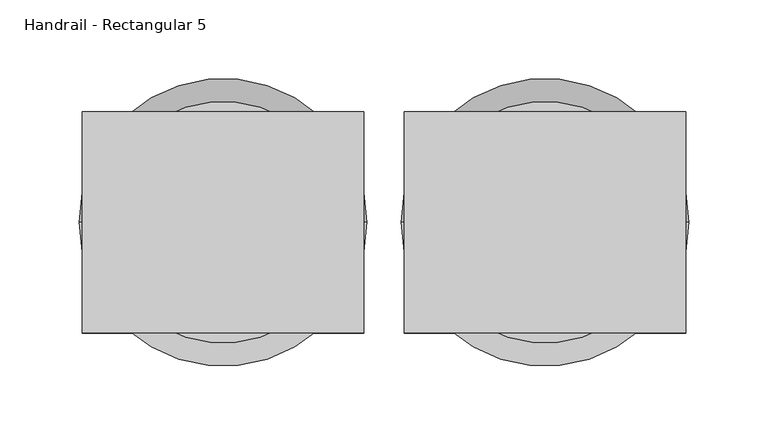
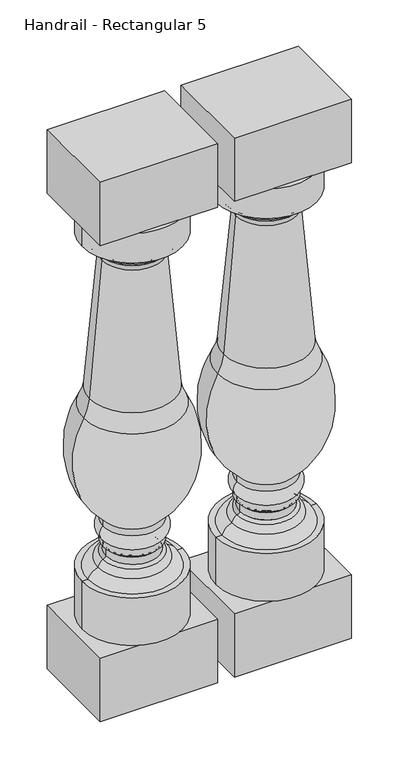
"""IFC4 building model written with IfcOpenShell, lengths in millimetres: railing geometry, Handrail - Rectangular 5."""

from ifc_helpers import new_model, si_unit, point, frame, origin, place, context, project, spatial, polyline, circle_curve, ellipse_curve, trimmed, outline, extrude, source, transform, mapped, element, save
from ifc_brep_helpers import plane_surface, cylinder_surface, revolved_surface, advanced_brep


def handrail_rectangular_5_87bace6c(model_context):
    return source(origin(), model_context, "Body", "SolidModel", [
        advanced_brep(
        [(16901.0521895, -1665.6164768, 873.125), (17053.4521895, -1665.6164768, 873.125), (16977.2521895, -1665.6164768, 873.125), (16901.0521895, -1665.6164768, 825.4490755), (17053.4521895, -1665.6164768, 825.4490755), (16911.0954208, -1665.6164768, 825.4490755), (17043.4089583, -1665.6164768, 825.4490755), (16922.5787107, -1665.6164768, 813.9657856), (17031.9256684, -1665.6164768, 813.9657856), (16922.5787107, -1665.6164768, 808.3461292), (17031.9256684, -1665.6164768, 808.3461292), (16928.2808978, -1665.6164768, 802.2016975), (17026.2234813, -1665.6164768, 802.2016975), (16931.6226936, -1665.6164768, 792.8428746), (17022.8816855, -1665.6164768, 792.8428746), (16912.8551876, -1665.6164768, 577.4758218), (17041.6491915, -1665.6164768, 577.4758218), (16903.837965, -1665.6164768, 549.5125844), (17050.6664141, -1665.6164768, 549.5125844), (16933.1087972, -1665.6164768, 376.7693301), (17021.3955818, -1665.6164768, 376.7693301), (16933.1087972, -1665.6164768, 366.4437154), (17021.3955818, -1665.6164768, 366.4437154), (16933.1087972, -1665.6164768, 343.8682651), (17021.3955818, -1665.6164768, 343.8682651), (16933.1087972, -1665.6164768, 333.5426504), (17021.3955818, -1665.6164768, 333.5426504), (16937.4192375, -1665.6164768, 329.2322102), (17017.0851416, -1665.6164768, 329.2322102), (16937.4192375, -1665.6164768, 317.4353211), (17017.0851416, -1665.6164768, 317.4353211), (16932.9214444, -1665.6164768, 313.1289544), (17021.5829347, -1665.6164768, 313.1289544), (16925.4009874, -1665.6164768, 303.0807869), (17029.1033917, -1665.6164768, 303.0807869), (16910.2523786, -1665.6164768, 288.925), (17044.2520004, -1665.6164768, 288.925), (16901.0521895, -1665.6164768, 288.925), (17053.4521895, -1665.6164768, 288.925), (16901.0521895, -1665.6164768, 212.725), (17053.4521895, -1665.6164768, 212.725), (16977.2521895, -1665.6164768, 212.725)],
        [
            (0, 1, circle_curve(frame((16977.2521895, -1665.6164768, 873.125), z_axis=(0.0, 0.0, 1.0), x_axis=(1.0, 0.0, 0.0)), 76.2)),
            (1, 2),
            (2, 0),
            (1, 0, circle_curve(frame((16977.2521895, -1665.6164768, 873.125), z_axis=(0.0, 0.0, 1.0), x_axis=(1.0, 0.0, 0.0)), 76.2)),
            (3, 4, circle_curve(frame((16977.2521895, -1665.6164768, 825.4490755), z_axis=(0.0, 0.0, 1.0), x_axis=(1.0, 0.0, 0.0)), 76.2)),
            (4, 1),
            (0, 3),
            (4, 3, circle_curve(frame((16977.2521895, -1665.6164768, 825.4490755), z_axis=(0.0, 0.0, 1.0), x_axis=(1.0, 0.0, 0.0)), 76.2)),
            (5, 6, circle_curve(frame((16977.2521895, -1665.6164768, 825.4490755), z_axis=(0.0, 0.0, 1.0), x_axis=(1.0, 0.0, 0.0)), 66.1567687)),
            (6, 4),
            (3, 5),
            (6, 5, circle_curve(frame((16977.2521895, -1665.6164768, 825.4490755), z_axis=(0.0, 0.0, 1.0), x_axis=(1.0, 0.0, 0.0)), 66.1567687)),
            (7, 8, circle_curve(frame((16977.2521895, -1665.6164768, 813.9657856), z_axis=(0.0, 0.0, 1.0), x_axis=(1.0, 0.0, 0.0)), 54.6734788)),
            (8, 6, circle_curve(frame((17031.9256684, -1665.6164768, 825.4490755), z_axis=(0.0, -1.0, 0.0), x_axis=(-1.0, 0.0, 0.0)), 11.4832899)),
            (5, 7, circle_curve(frame((16922.5787107, -1665.6164768, 825.4490755), z_axis=(0.0, -1.0, 0.0), x_axis=(1.0, 0.0, 0.0)), 11.4832899)),
            (8, 7, circle_curve(frame((16977.2521895, -1665.6164768, 813.9657856), z_axis=(0.0, 0.0, 1.0), x_axis=(1.0, 0.0, 0.0)), 54.6734788)),
            (9, 10, circle_curve(frame((16977.2521895, -1665.6164768, 808.3461292), z_axis=(0.0, 0.0, 1.0), x_axis=(1.0, 0.0, 0.0)), 54.6734788)),
            (10, 8),
            (7, 9),
            (10, 9, circle_curve(frame((16977.2521895, -1665.6164768, 808.3461292), z_axis=(0.0, 0.0, 1.0), x_axis=(1.0, 0.0, 0.0)), 54.6734788)),
            (11, 12, circle_curve(frame((16977.2521895, -1665.6164768, 802.2016975), z_axis=(0.0, 0.0, 1.0), x_axis=(1.0, 0.0, 0.0)), 48.9712918)),
            (12, 10, circle_curve(frame((17039.6345288, -1665.6164768, 795.4740105), z_axis=(0.0, 1.0, 0.0), x_axis=(-1.0, 0.0, 0.0)), 15.0039317)),
            (9, 11, circle_curve(frame((16914.8698503, -1665.6164768, 795.4740105), z_axis=(0.0, 1.0, 0.0), x_axis=(1.0, 0.0, 0.0)), 15.0039317)),
            (12, 11, circle_curve(frame((16977.2521895, -1665.6164768, 802.2016975), z_axis=(0.0, 0.0, 1.0), x_axis=(1.0, 0.0, 0.0)), 48.9712918)),
            (13, 14, circle_curve(frame((16977.2521895, -1665.6164768, 792.8428746), z_axis=(0.0, 0.0, 1.0), x_axis=(1.0, 0.0, 0.0)), 45.629496)),
            (14, 12, circle_curve(frame((17035.5595739, -1665.6164768, 793.5919719), z_axis=(0.0, 1.0, 0.0), x_axis=(-1.0, 0.0, 0.0)), 12.7)),
            (11, 13, circle_curve(frame((16918.9448052, -1665.6164768, 793.5919719), z_axis=(0.0, 1.0, 0.0), x_axis=(1.0, 0.0, 0.0)), 12.7)),
            (14, 13, circle_curve(frame((16977.2521895, -1665.6164768, 792.8428746), z_axis=(0.0, 0.0, 1.0), x_axis=(1.0, 0.0, 0.0)), 45.629496)),
            (15, 16, circle_curve(frame((16977.2521895, -1665.6164768, 577.4758218), z_axis=(0.0, 0.0, 1.0), x_axis=(1.0, 0.0, 0.0)), 64.3970019)),
            (16, 14, circle_curve(frame((20890.3232099, -1665.6164768, 1021.358044), z_axis=(0.0, 1.0, 0.0), x_axis=(-1.0, 0.0, 0.0)), 3874.1867698)),
            (13, 15, circle_curve(frame((13064.1811691, -1665.6164768, 1021.358044), z_axis=(0.0, 1.0, 0.0), x_axis=(1.0, 0.0, 0.0)), 3874.1867698)),
            (16, 15, circle_curve(frame((16977.2521895, -1665.6164768, 577.4758218), z_axis=(0.0, 0.0, 1.0), x_axis=(1.0, 0.0, 0.0)), 64.3970019)),
            (17, 18, circle_curve(frame((16977.2521895, -1665.6164768, 549.5125844), z_axis=(0.0, 0.0, 1.0), x_axis=(1.0, 0.0, 0.0)), 73.4142246)),
            (18, 16, circle_curve(frame((17116.1688441, -1665.6164768, 586.070457), z_axis=(0.0, 1.0, 0.0), x_axis=(-1.0, 0.0, 0.0)), 75.0136413)),
            (15, 17, circle_curve(frame((16838.335535, -1665.6164768, 586.070457), z_axis=(0.0, 1.0, 0.0), x_axis=(1.0, 0.0, 0.0)), 75.0136413)),
            (18, 17, circle_curve(frame((16977.2521895, -1665.6164768, 549.5125844), z_axis=(0.0, 0.0, 1.0), x_axis=(1.0, 0.0, 0.0)), 73.4142246)),
            (19, 20, circle_curve(frame((16977.2521895, -1665.6164768, 376.7693301), z_axis=(0.0, 0.0, 1.0), x_axis=(1.0, 0.0, 0.0)), 44.1433923)),
            (20, 18, circle_curve(frame((16928.5440648, -1665.6164768, 481.3542994), z_axis=(0.0, -1.0, 0.0), x_axis=(-1.0, 0.0, 0.0)), 139.8549964)),
            (17, 19, circle_curve(frame((17025.9603143, -1665.6164768, 481.3542994), z_axis=(0.0, -1.0, 0.0), x_axis=(1.0, 0.0, 0.0)), 139.8549964)),
            (20, 19, circle_curve(frame((16977.2521895, -1665.6164768, 376.7693301), z_axis=(0.0, 0.0, 1.0), x_axis=(1.0, 0.0, 0.0)), 44.1433923)),
            (21, 22, circle_curve(frame((16977.2521895, -1665.6164768, 366.4437154), z_axis=(0.0, 0.0, 1.0), x_axis=(1.0, 0.0, 0.0)), 44.1433923)),
            (22, 20),
            (19, 21),
            (22, 21, circle_curve(frame((16977.2521895, -1665.6164768, 366.4437154), z_axis=(0.0, 0.0, 1.0), x_axis=(1.0, 0.0, 0.0)), 44.1433923)),
            (23, 24, circle_curve(frame((16977.2521895, -1665.6164768, 343.8682651), z_axis=(0.0, 0.0, 1.0), x_axis=(1.0, 0.0, 0.0)), 44.1433923)),
            (24, 22, circle_curve(frame((17013.103554, -1665.6164768, 355.1559903), z_axis=(0.0, -1.0, 0.0), x_axis=(-1.0, 0.0, 0.0)), 14.0060867)),
            (21, 23, circle_curve(frame((16941.4008251, -1665.6164768, 355.1559903), z_axis=(0.0, -1.0, 0.0), x_axis=(1.0, 0.0, 0.0)), 14.0060867)),
            (24, 23, circle_curve(frame((16977.2521895, -1665.6164768, 343.8682651), z_axis=(0.0, 0.0, 1.0), x_axis=(1.0, 0.0, 0.0)), 44.1433923)),
            (25, 26, circle_curve(frame((16977.2521895, -1665.6164768, 333.5426504), z_axis=(0.0, 0.0, 1.0), x_axis=(1.0, 0.0, 0.0)), 44.1433923)),
            (26, 24),
            (23, 25),
            (26, 25, circle_curve(frame((16977.2521895, -1665.6164768, 333.5426504), z_axis=(0.0, 0.0, 1.0), x_axis=(1.0, 0.0, 0.0)), 44.1433923)),
            (27, 28, circle_curve(frame((16977.2521895, -1665.6164768, 329.2322102), z_axis=(0.0, 0.0, 1.0), x_axis=(1.0, 0.0, 0.0)), 39.8329521)),
            (28, 26, circle_curve(frame((17021.3955818, -1665.6164768, 329.2322102), z_axis=(0.0, 1.0, 0.0), x_axis=(-1.0, 0.0, 0.0)), 4.3104402)),
            (25, 27, circle_curve(frame((16933.1087972, -1665.6164768, 329.2322102), z_axis=(0.0, 1.0, 0.0), x_axis=(1.0, 0.0, 0.0)), 4.3104402)),
            (28, 27, circle_curve(frame((16977.2521895, -1665.6164768, 329.2322102), z_axis=(0.0, 0.0, 1.0), x_axis=(1.0, 0.0, 0.0)), 39.8329521)),
            (29, 30, circle_curve(frame((16977.2521895, -1665.6164768, 317.4353211), z_axis=(0.0, 0.0, 1.0), x_axis=(1.0, 0.0, 0.0)), 39.8329521)),
            (30, 28),
            (27, 29),
            (30, 29, circle_curve(frame((16977.2521895, -1665.6164768, 317.4353211), z_axis=(0.0, 0.0, 1.0), x_axis=(1.0, 0.0, 0.0)), 39.8329521)),
            (31, 32, circle_curve(frame((16977.2521895, -1665.6164768, 313.1289544), z_axis=(0.0, 0.0, 1.0), x_axis=(1.0, 0.0, 0.0)), 44.3307451)),
            (32, 30, circle_curve(frame((17021.3955818, -1665.6164768, 317.4353211), z_axis=(0.0, 1.0, 0.0), x_axis=(-1.0, 0.0, 0.0)), 4.3104402)),
            (29, 31, circle_curve(frame((16933.1087972, -1665.6164768, 317.4353211), z_axis=(0.0, 1.0, 0.0), x_axis=(1.0, 0.0, 0.0)), 4.3104402)),
            (32, 31, circle_curve(frame((16977.2521895, -1665.6164768, 313.1289544), z_axis=(0.0, 0.0, 1.0), x_axis=(1.0, 0.0, 0.0)), 44.3307451)),
            (33, 34, circle_curve(frame((16977.2521895, -1665.6164768, 303.0807869), z_axis=(0.0, 0.0, 1.0), x_axis=(1.0, 0.0, 0.0)), 51.8512022)),
            (34, 32, circle_curve(frame((17014.4640754, -1665.6164768, 299.962519), z_axis=(0.0, -1.0, 0.0), x_axis=(-1.0, 0.0, 0.0)), 14.9677378)),
            (31, 33, circle_curve(frame((16940.0403037, -1665.6164768, 299.962519), z_axis=(0.0, -1.0, 0.0), x_axis=(1.0, 0.0, 0.0)), 14.9677378)),
            (34, 33, circle_curve(frame((16977.2521895, -1665.6164768, 303.0807869), z_axis=(0.0, 0.0, 1.0), x_axis=(1.0, 0.0, 0.0)), 51.8512022)),
            (35, 36, circle_curve(frame((16977.2521895, -1665.6164768, 288.925), z_axis=(0.0, 0.0, 1.0), x_axis=(1.0, 0.0, 0.0)), 66.9998109)),
            (36, 34, circle_curve(frame((17023.8545436, -1665.6164768, 282.2803841), z_axis=(0.0, -1.0, 0.0), x_axis=(-1.0, 0.0, 0.0)), 21.4524396)),
            (33, 35, circle_curve(frame((16930.6498354, -1665.6164768, 282.2803841), z_axis=(0.0, -1.0, 0.0), x_axis=(1.0, 0.0, 0.0)), 21.4524396)),
            (36, 35, circle_curve(frame((16977.2521895, -1665.6164768, 288.925), z_axis=(0.0, 0.0, 1.0), x_axis=(1.0, 0.0, 0.0)), 66.9998109)),
            (37, 38, circle_curve(frame((16977.2521895, -1665.6164768, 288.925), z_axis=(0.0, 0.0, 1.0), x_axis=(1.0, 0.0, 0.0)), 76.2)),
            (38, 36),
            (35, 37),
            (38, 37, circle_curve(frame((16977.2521895, -1665.6164768, 288.925), z_axis=(0.0, 0.0, 1.0), x_axis=(1.0, 0.0, 0.0)), 76.2)),
            (39, 40, circle_curve(frame((16977.2521895, -1665.6164768, 212.725), z_axis=(0.0, 0.0, 1.0), x_axis=(1.0, 0.0, 0.0)), 76.2)),
            (40, 38),
            (37, 39),
            (40, 39, circle_curve(frame((16977.2521895, -1665.6164768, 212.725), z_axis=(0.0, 0.0, 1.0), x_axis=(1.0, 0.0, 0.0)), 76.2)),
            (41, 40),
            (39, 41),
        ],
        [
            plane_surface(frame((16977.2521895, -1665.6164768, 873.125), z_axis=(0.0, 0.0, 1.0), x_axis=(1.0, 0.0, 0.0))),
            cylinder_surface(frame((16977.2521895, -1665.6164768, 841.375), z_axis=(0.0, 0.0, -1.0), x_axis=(1.0, 0.0, 0.0)), 76.2),
            plane_surface(frame((16977.2521895, -1665.6164768, 825.4490755), z_axis=(0.0, 0.0, -1.0), x_axis=(1.0, 0.0, 0.0))),
            revolved_surface(trimmed(ellipse_curve(frame((17031.9256684, -1665.6164768, 825.4490755), z_axis=(0.0, 1.0, 0.0), x_axis=(-1.0, 0.0, 0.0)), 11.4832899, 11.4832899), [point((17043.4089583, -1665.6164768, 825.4490755))], [point((17031.9256684, -1665.6164768, 813.9657856))], True, "CARTESIAN"), (16977.2521895, -1665.6164768, 841.375), (0.0, 0.0, -1.0)),
            cylinder_surface(frame((16977.2521895, -1665.6164768, 841.375), z_axis=(0.0, 0.0, -1.0), x_axis=(1.0, 0.0, 0.0)), 54.6734788),
            revolved_surface(trimmed(ellipse_curve(frame((17039.6345288, -1665.6164768, 795.4740105), z_axis=(0.0, -1.0, 0.0), x_axis=(-1.0, 0.0, 0.0)), 15.0039317, 15.0039317), [point((17031.9256684, -1665.6164768, 808.3461292))], [point((17026.2234813, -1665.6164768, 802.2016975))], True, "CARTESIAN"), (16977.2521895, -1665.6164768, 841.375), (0.0, 0.0, -1.0)),
            revolved_surface(trimmed(ellipse_curve(frame((17035.5595739, -1665.6164768, 793.5919719), z_axis=(0.0, -1.0, 0.0), x_axis=(-1.0, 0.0, 0.0)), 12.7, 12.7), [point((17026.2234813, -1665.6164768, 802.2016975))], [point((17022.8816855, -1665.6164768, 792.8428746))], True, "CARTESIAN"), (16977.2521895, -1665.6164768, 841.375), (0.0, 0.0, -1.0)),
            revolved_surface(trimmed(ellipse_curve(frame((20890.3232099, -1665.6164768, 1021.358044), z_axis=(0.0, -1.0, 0.0), x_axis=(-1.0, 0.0, 0.0)), 3874.1867698, 3874.1867698), [point((17022.8816855, -1665.6164768, 792.8428746))], [point((17041.6491915, -1665.6164768, 577.4758218))], True, "CARTESIAN"), (16977.2521895, -1665.6164768, 841.375), (0.0, 0.0, -1.0)),
            revolved_surface(trimmed(ellipse_curve(frame((17116.1688441, -1665.6164768, 586.070457), z_axis=(0.0, -1.0, 0.0), x_axis=(-1.0, 0.0, 0.0)), 75.0136413, 75.0136413), [point((17041.6491915, -1665.6164768, 577.4758218))], [point((17050.6664141, -1665.6164768, 549.5125844))], True, "CARTESIAN"), (16977.2521895, -1665.6164768, 841.375), (0.0, 0.0, -1.0)),
            revolved_surface(trimmed(ellipse_curve(frame((16928.5440648, -1665.6164768, 481.3542994), z_axis=(0.0, 1.0, 0.0), x_axis=(-1.0, 0.0, 0.0)), 139.8549964, 139.8549964), [point((17050.6664141, -1665.6164768, 549.5125844))], [point((17021.3955818, -1665.6164768, 376.7693301))], True, "CARTESIAN"), (16977.2521895, -1665.6164768, 841.375), (0.0, 0.0, -1.0)),
            cylinder_surface(frame((16977.2521895, -1665.6164768, 841.375), z_axis=(0.0, 0.0, -1.0), x_axis=(1.0, 0.0, 0.0)), 44.1433923),
            revolved_surface(trimmed(ellipse_curve(frame((17013.103554, -1665.6164768, 355.1559903), z_axis=(0.0, 1.0, 0.0), x_axis=(-1.0, 0.0, 0.0)), 14.0060867, 14.0060867), [point((17021.3955818, -1665.6164768, 366.4437154))], [point((17021.3955818, -1665.6164768, 343.8682651))], True, "CARTESIAN"), (16977.2521895, -1665.6164768, 841.375), (0.0, 0.0, -1.0)),
            revolved_surface(trimmed(ellipse_curve(frame((17021.3955818, -1665.6164768, 329.2322102), z_axis=(0.0, -1.0, 0.0), x_axis=(-1.0, 0.0, 0.0)), 4.3104402, 4.3104402), [point((17021.3955818, -1665.6164768, 333.5426504))], [point((17017.0851416, -1665.6164768, 329.2322102))], True, "CARTESIAN"), (16977.2521895, -1665.6164768, 841.375), (0.0, 0.0, -1.0)),
            cylinder_surface(frame((16977.2521895, -1665.6164768, 841.375), z_axis=(0.0, 0.0, -1.0), x_axis=(1.0, 0.0, 0.0)), 39.8329521),
            revolved_surface(trimmed(ellipse_curve(frame((17021.3955818, -1665.6164768, 317.4353211), z_axis=(0.0, -1.0, 0.0), x_axis=(-1.0, 0.0, 0.0)), 4.3104402, 4.3104402), [point((17017.0851416, -1665.6164768, 317.4353211))], [point((17021.5829347, -1665.6164768, 313.1289544))], True, "CARTESIAN"), (16977.2521895, -1665.6164768, 841.375), (0.0, 0.0, -1.0)),
            revolved_surface(trimmed(ellipse_curve(frame((17014.4640754, -1665.6164768, 299.962519), z_axis=(0.0, 1.0, 0.0), x_axis=(-1.0, 0.0, 0.0)), 14.9677378, 14.9677378), [point((17021.5829347, -1665.6164768, 313.1289544))], [point((17029.1033917, -1665.6164768, 303.0807869))], True, "CARTESIAN"), (16977.2521895, -1665.6164768, 841.375), (0.0, 0.0, -1.0)),
            revolved_surface(trimmed(ellipse_curve(frame((17023.8545436, -1665.6164768, 282.2803841), z_axis=(0.0, 1.0, 0.0), x_axis=(-1.0, 0.0, 0.0)), 21.4524396, 21.4524396), [point((17029.1033917, -1665.6164768, 303.0807869))], [point((17044.2520004, -1665.6164768, 288.925))], True, "CARTESIAN"), (16977.2521895, -1665.6164768, 841.375), (0.0, 0.0, -1.0)),
            plane_surface(frame((16977.2521895, -1665.6164768, 288.925), z_axis=(0.0, 0.0, 1.0), x_axis=(1.0, 0.0, 0.0))),
            plane_surface(frame((16977.2521895, -1665.6164768, 212.725), z_axis=(0.0, 0.0, -1.0), x_axis=(1.0, 0.0, 0.0))),
        ],
        [
            (0, [[1, 2, 3]]),
            (0, [[4, -3, -2]]),
            (1, [[5, 6, -1, 7]]),
            (1, [[8, -7, -4, -6]]),
            (2, [[9, 10, -5, 11]]),
            (2, [[12, -11, -8, -10]]),
            (3, [[13, 14, -9, 15]]),
            (3, [[16, -15, -12, -14]]),
            (4, [[17, 18, -13, 19]]),
            (4, [[20, -19, -16, -18]]),
            (5, [[21, 22, -17, 23]]),
            (5, [[24, -23, -20, -22]]),
            (6, [[25, 26, -21, 27]]),
            (6, [[28, -27, -24, -26]]),
            (7, [[29, 30, -25, 31]]),
            (7, [[32, -31, -28, -30]]),
            (8, [[33, 34, -29, 35]]),
            (8, [[36, -35, -32, -34]]),
            (9, [[37, 38, -33, 39]]),
            (9, [[40, -39, -36, -38]]),
            (10, [[41, 42, -37, 43]]),
            (10, [[44, -43, -40, -42]]),
            (11, [[45, 46, -41, 47]]),
            (11, [[48, -47, -44, -46]]),
            (10, [[49, 50, -45, 51]]),
            (10, [[52, -51, -48, -50]]),
            (12, [[53, 54, -49, 55]]),
            (12, [[56, -55, -52, -54]]),
            (13, [[57, 58, -53, 59]]),
            (13, [[60, -59, -56, -58]]),
            (14, [[61, 62, -57, 63]]),
            (14, [[64, -63, -60, -62]]),
            (15, [[65, 66, -61, 67]]),
            (15, [[68, -67, -64, -66]]),
            (16, [[69, 70, -65, 71]]),
            (16, [[72, -71, -68, -70]]),
            (17, [[73, 74, -69, 75]]),
            (17, [[76, -75, -72, -74]]),
            (1, [[77, 78, -73, 79]]),
            (1, [[80, -79, -76, -78]]),
            (18, [[81, -77, 82]]),
            (18, [[-82, -80, -81]]),
        ],
    ),
        extrude(outline(polyline([(16888.3521895, -1735.4664768), (16888.3521895, -1595.7664768), (17066.1521895, -1595.7664768), (17066.1521895, -1735.4664768), (16888.3521895, -1735.4664768)])), frame((0.0, 0.0, 111.125), z_axis=(0.0, 0.0, 1.0), x_axis=(1.0, 0.0, 0.0)), (0.0, 0.0, 1.0), 101.6),
        extrude(outline(polyline([(16888.3521895, -1595.7664768), (17066.1521895, -1595.7664768), (17066.1521895, -1735.4664768), (16888.3521895, -1735.4664768), (16888.3521895, -1595.7664768)])), frame((0.0, 0.0, 873.125), z_axis=(0.0, 0.0, 1.0), x_axis=(1.0, 0.0, 0.0)), (0.0, 0.0, 1.0), 101.6),
        advanced_brep(
        [(16697.8521895, -1665.6164768, 873.125), (16850.2521895, -1665.6164768, 873.125), (16774.0521895, -1665.6164768, 873.125), (16697.8521895, -1665.6164768, 825.4490755), (16850.2521895, -1665.6164768, 825.4490755), (16707.8954208, -1665.6164768, 825.4490755), (16840.2089583, -1665.6164768, 825.4490755), (16719.3787107, -1665.6164768, 813.9657856), (16828.7256684, -1665.6164768, 813.9657856), (16719.3787107, -1665.6164768, 808.3461292), (16828.7256684, -1665.6164768, 808.3461292), (16725.0808978, -1665.6164768, 802.2016975), (16823.0234813, -1665.6164768, 802.2016975), (16728.4226936, -1665.6164768, 792.8428746), (16819.6816855, -1665.6164768, 792.8428746), (16709.6551876, -1665.6164768, 577.4758218), (16838.4491915, -1665.6164768, 577.4758218), (16700.637965, -1665.6164768, 549.5125844), (16847.4664141, -1665.6164768, 549.5125844), (16729.9087972, -1665.6164768, 376.7693301), (16818.1955818, -1665.6164768, 376.7693301), (16729.9087972, -1665.6164768, 366.4437154), (16818.1955818, -1665.6164768, 366.4437154), (16729.9087972, -1665.6164768, 343.8682651), (16818.1955818, -1665.6164768, 343.8682651), (16729.9087972, -1665.6164768, 333.5426504), (16818.1955818, -1665.6164768, 333.5426504), (16734.2192375, -1665.6164768, 329.2322102), (16813.8851416, -1665.6164768, 329.2322102), (16734.2192375, -1665.6164768, 317.4353211), (16813.8851416, -1665.6164768, 317.4353211), (16729.7214444, -1665.6164768, 313.1289544), (16818.3829347, -1665.6164768, 313.1289544), (16722.2009874, -1665.6164768, 303.0807869), (16825.9033917, -1665.6164768, 303.0807869), (16707.0523786, -1665.6164768, 288.925), (16841.0520004, -1665.6164768, 288.925), (16697.8521895, -1665.6164768, 288.925), (16850.2521895, -1665.6164768, 288.925), (16697.8521895, -1665.6164768, 212.725), (16850.2521895, -1665.6164768, 212.725), (16774.0521895, -1665.6164768, 212.725)],
        [
            (0, 1, circle_curve(frame((16774.0521895, -1665.6164768, 873.125), z_axis=(0.0, 0.0, 1.0), x_axis=(1.0, 0.0, 0.0)), 76.2)),
            (1, 2),
            (2, 0),
            (1, 0, circle_curve(frame((16774.0521895, -1665.6164768, 873.125), z_axis=(0.0, 0.0, 1.0), x_axis=(1.0, 0.0, 0.0)), 76.2)),
            (3, 4, circle_curve(frame((16774.0521895, -1665.6164768, 825.4490755), z_axis=(0.0, 0.0, 1.0), x_axis=(1.0, 0.0, 0.0)), 76.2)),
            (4, 1),
            (0, 3),
            (4, 3, circle_curve(frame((16774.0521895, -1665.6164768, 825.4490755), z_axis=(0.0, 0.0, 1.0), x_axis=(1.0, 0.0, 0.0)), 76.2)),
            (5, 6, circle_curve(frame((16774.0521895, -1665.6164768, 825.4490755), z_axis=(0.0, 0.0, 1.0), x_axis=(1.0, 0.0, 0.0)), 66.1567687)),
            (6, 4),
            (3, 5),
            (6, 5, circle_curve(frame((16774.0521895, -1665.6164768, 825.4490755), z_axis=(0.0, 0.0, 1.0), x_axis=(1.0, 0.0, 0.0)), 66.1567687)),
            (7, 8, circle_curve(frame((16774.0521895, -1665.6164768, 813.9657856), z_axis=(0.0, 0.0, 1.0), x_axis=(1.0, 0.0, 0.0)), 54.6734788)),
            (8, 6, circle_curve(frame((16828.7256684, -1665.6164768, 825.4490755), z_axis=(0.0, -1.0, 0.0), x_axis=(-1.0, 0.0, 0.0)), 11.4832899)),
            (5, 7, circle_curve(frame((16719.3787107, -1665.6164768, 825.4490755), z_axis=(0.0, -1.0, 0.0), x_axis=(1.0, 0.0, 0.0)), 11.4832899)),
            (8, 7, circle_curve(frame((16774.0521895, -1665.6164768, 813.9657856), z_axis=(0.0, 0.0, 1.0), x_axis=(1.0, 0.0, 0.0)), 54.6734788)),
            (9, 10, circle_curve(frame((16774.0521895, -1665.6164768, 808.3461292), z_axis=(0.0, 0.0, 1.0), x_axis=(1.0, 0.0, 0.0)), 54.6734788)),
            (10, 8),
            (7, 9),
            (10, 9, circle_curve(frame((16774.0521895, -1665.6164768, 808.3461292), z_axis=(0.0, 0.0, 1.0), x_axis=(1.0, 0.0, 0.0)), 54.6734788)),
            (11, 12, circle_curve(frame((16774.0521895, -1665.6164768, 802.2016975), z_axis=(0.0, 0.0, 1.0), x_axis=(1.0, 0.0, 0.0)), 48.9712918)),
            (12, 10, circle_curve(frame((16836.4345288, -1665.6164768, 795.4740105), z_axis=(0.0, 1.0, 0.0), x_axis=(-1.0, 0.0, 0.0)), 15.0039317)),
            (9, 11, circle_curve(frame((16711.6698503, -1665.6164768, 795.4740105), z_axis=(0.0, 1.0, 0.0), x_axis=(1.0, 0.0, 0.0)), 15.0039317)),
            (12, 11, circle_curve(frame((16774.0521895, -1665.6164768, 802.2016975), z_axis=(0.0, 0.0, 1.0), x_axis=(1.0, 0.0, 0.0)), 48.9712918)),
            (13, 14, circle_curve(frame((16774.0521895, -1665.6164768, 792.8428746), z_axis=(0.0, 0.0, 1.0), x_axis=(1.0, 0.0, 0.0)), 45.629496)),
            (14, 12, circle_curve(frame((16832.3595739, -1665.6164768, 793.5919719), z_axis=(0.0, 1.0, 0.0), x_axis=(-1.0, 0.0, 0.0)), 12.7)),
            (11, 13, circle_curve(frame((16715.7448052, -1665.6164768, 793.5919719), z_axis=(0.0, 1.0, 0.0), x_axis=(1.0, 0.0, 0.0)), 12.7)),
            (14, 13, circle_curve(frame((16774.0521895, -1665.6164768, 792.8428746), z_axis=(0.0, 0.0, 1.0), x_axis=(1.0, 0.0, 0.0)), 45.629496)),
            (15, 16, circle_curve(frame((16774.0521895, -1665.6164768, 577.4758218), z_axis=(0.0, 0.0, 1.0), x_axis=(1.0, 0.0, 0.0)), 64.3970019)),
            (16, 14, circle_curve(frame((20687.1232099, -1665.6164768, 1021.358044), z_axis=(0.0, 1.0, 0.0), x_axis=(-1.0, 0.0, 0.0)), 3874.1867698)),
            (13, 15, circle_curve(frame((12860.9811691, -1665.6164768, 1021.358044), z_axis=(0.0, 1.0, 0.0), x_axis=(1.0, 0.0, 0.0)), 3874.1867698)),
            (16, 15, circle_curve(frame((16774.0521895, -1665.6164768, 577.4758218), z_axis=(0.0, 0.0, 1.0), x_axis=(1.0, 0.0, 0.0)), 64.3970019)),
            (17, 18, circle_curve(frame((16774.0521895, -1665.6164768, 549.5125844), z_axis=(0.0, 0.0, 1.0), x_axis=(1.0, 0.0, 0.0)), 73.4142246)),
            (18, 16, circle_curve(frame((16912.9688441, -1665.6164768, 586.070457), z_axis=(0.0, 1.0, 0.0), x_axis=(-1.0, 0.0, 0.0)), 75.0136413)),
            (15, 17, circle_curve(frame((16635.135535, -1665.6164768, 586.070457), z_axis=(0.0, 1.0, 0.0), x_axis=(1.0, 0.0, 0.0)), 75.0136413)),
            (18, 17, circle_curve(frame((16774.0521895, -1665.6164768, 549.5125844), z_axis=(0.0, 0.0, 1.0), x_axis=(1.0, 0.0, 0.0)), 73.4142246)),
            (19, 20, circle_curve(frame((16774.0521895, -1665.6164768, 376.7693301), z_axis=(0.0, 0.0, 1.0), x_axis=(1.0, 0.0, 0.0)), 44.1433923)),
            (20, 18, circle_curve(frame((16725.3440648, -1665.6164768, 481.3542994), z_axis=(0.0, -1.0, 0.0), x_axis=(-1.0, 0.0, 0.0)), 139.8549964)),
            (17, 19, circle_curve(frame((16822.7603143, -1665.6164768, 481.3542994), z_axis=(0.0, -1.0, 0.0), x_axis=(1.0, 0.0, 0.0)), 139.8549964)),
            (20, 19, circle_curve(frame((16774.0521895, -1665.6164768, 376.7693301), z_axis=(0.0, 0.0, 1.0), x_axis=(1.0, 0.0, 0.0)), 44.1433923)),
            (21, 22, circle_curve(frame((16774.0521895, -1665.6164768, 366.4437154), z_axis=(0.0, 0.0, 1.0), x_axis=(1.0, 0.0, 0.0)), 44.1433923)),
            (22, 20),
            (19, 21),
            (22, 21, circle_curve(frame((16774.0521895, -1665.6164768, 366.4437154), z_axis=(0.0, 0.0, 1.0), x_axis=(1.0, 0.0, 0.0)), 44.1433923)),
            (23, 24, circle_curve(frame((16774.0521895, -1665.6164768, 343.8682651), z_axis=(0.0, 0.0, 1.0), x_axis=(1.0, 0.0, 0.0)), 44.1433923)),
            (24, 22, circle_curve(frame((16809.903554, -1665.6164768, 355.1559903), z_axis=(0.0, -1.0, 0.0), x_axis=(-1.0, 0.0, 0.0)), 14.0060867)),
            (21, 23, circle_curve(frame((16738.2008251, -1665.6164768, 355.1559903), z_axis=(0.0, -1.0, 0.0), x_axis=(1.0, 0.0, 0.0)), 14.0060867)),
            (24, 23, circle_curve(frame((16774.0521895, -1665.6164768, 343.8682651), z_axis=(0.0, 0.0, 1.0), x_axis=(1.0, 0.0, 0.0)), 44.1433923)),
            (25, 26, circle_curve(frame((16774.0521895, -1665.6164768, 333.5426504), z_axis=(0.0, 0.0, 1.0), x_axis=(1.0, 0.0, 0.0)), 44.1433923)),
            (26, 24),
            (23, 25),
            (26, 25, circle_curve(frame((16774.0521895, -1665.6164768, 333.5426504), z_axis=(0.0, 0.0, 1.0), x_axis=(1.0, 0.0, 0.0)), 44.1433923)),
            (27, 28, circle_curve(frame((16774.0521895, -1665.6164768, 329.2322102), z_axis=(0.0, 0.0, 1.0), x_axis=(1.0, 0.0, 0.0)), 39.8329521)),
            (28, 26, circle_curve(frame((16818.1955818, -1665.6164768, 329.2322102), z_axis=(0.0, 1.0, 0.0), x_axis=(-1.0, 0.0, 0.0)), 4.3104402)),
            (25, 27, circle_curve(frame((16729.9087972, -1665.6164768, 329.2322102), z_axis=(0.0, 1.0, 0.0), x_axis=(1.0, 0.0, 0.0)), 4.3104402)),
            (28, 27, circle_curve(frame((16774.0521895, -1665.6164768, 329.2322102), z_axis=(0.0, 0.0, 1.0), x_axis=(1.0, 0.0, 0.0)), 39.8329521)),
            (29, 30, circle_curve(frame((16774.0521895, -1665.6164768, 317.4353211), z_axis=(0.0, 0.0, 1.0), x_axis=(1.0, 0.0, 0.0)), 39.8329521)),
            (30, 28),
            (27, 29),
            (30, 29, circle_curve(frame((16774.0521895, -1665.6164768, 317.4353211), z_axis=(0.0, 0.0, 1.0), x_axis=(1.0, 0.0, 0.0)), 39.8329521)),
            (31, 32, circle_curve(frame((16774.0521895, -1665.6164768, 313.1289544), z_axis=(0.0, 0.0, 1.0), x_axis=(1.0, 0.0, 0.0)), 44.3307451)),
            (32, 30, circle_curve(frame((16818.1955818, -1665.6164768, 317.4353211), z_axis=(0.0, 1.0, 0.0), x_axis=(-1.0, 0.0, 0.0)), 4.3104402)),
            (29, 31, circle_curve(frame((16729.9087972, -1665.6164768, 317.4353211), z_axis=(0.0, 1.0, 0.0), x_axis=(1.0, 0.0, 0.0)), 4.3104402)),
            (32, 31, circle_curve(frame((16774.0521895, -1665.6164768, 313.1289544), z_axis=(0.0, 0.0, 1.0), x_axis=(1.0, 0.0, 0.0)), 44.3307451)),
            (33, 34, circle_curve(frame((16774.0521895, -1665.6164768, 303.0807869), z_axis=(0.0, 0.0, 1.0), x_axis=(1.0, 0.0, 0.0)), 51.8512022)),
            (34, 32, circle_curve(frame((16811.2640754, -1665.6164768, 299.962519), z_axis=(0.0, -1.0, 0.0), x_axis=(-1.0, 0.0, 0.0)), 14.9677378)),
            (31, 33, circle_curve(frame((16736.8403037, -1665.6164768, 299.962519), z_axis=(0.0, -1.0, 0.0), x_axis=(1.0, 0.0, 0.0)), 14.9677378)),
            (34, 33, circle_curve(frame((16774.0521895, -1665.6164768, 303.0807869), z_axis=(0.0, 0.0, 1.0), x_axis=(1.0, 0.0, 0.0)), 51.8512022)),
            (35, 36, circle_curve(frame((16774.0521895, -1665.6164768, 288.925), z_axis=(0.0, 0.0, 1.0), x_axis=(1.0, 0.0, 0.0)), 66.9998109)),
            (36, 34, circle_curve(frame((16820.6545436, -1665.6164768, 282.2803841), z_axis=(0.0, -1.0, 0.0), x_axis=(-1.0, 0.0, 0.0)), 21.4524396)),
            (33, 35, circle_curve(frame((16727.4498354, -1665.6164768, 282.2803841), z_axis=(0.0, -1.0, 0.0), x_axis=(1.0, 0.0, 0.0)), 21.4524396)),
            (36, 35, circle_curve(frame((16774.0521895, -1665.6164768, 288.925), z_axis=(0.0, 0.0, 1.0), x_axis=(1.0, 0.0, 0.0)), 66.9998109)),
            (37, 38, circle_curve(frame((16774.0521895, -1665.6164768, 288.925), z_axis=(0.0, 0.0, 1.0), x_axis=(1.0, 0.0, 0.0)), 76.2)),
            (38, 36),
            (35, 37),
            (38, 37, circle_curve(frame((16774.0521895, -1665.6164768, 288.925), z_axis=(0.0, 0.0, 1.0), x_axis=(1.0, 0.0, 0.0)), 76.2)),
            (39, 40, circle_curve(frame((16774.0521895, -1665.6164768, 212.725), z_axis=(0.0, 0.0, 1.0), x_axis=(1.0, 0.0, 0.0)), 76.2)),
            (40, 38),
            (37, 39),
            (40, 39, circle_curve(frame((16774.0521895, -1665.6164768, 212.725), z_axis=(0.0, 0.0, 1.0), x_axis=(1.0, 0.0, 0.0)), 76.2)),
            (41, 40),
            (39, 41),
        ],
        [
            plane_surface(frame((16774.0521895, -1665.6164768, 873.125), z_axis=(0.0, 0.0, 1.0), x_axis=(1.0, 0.0, 0.0))),
            cylinder_surface(frame((16774.0521895, -1665.6164768, 841.375), z_axis=(0.0, 0.0, -1.0), x_axis=(1.0, 0.0, 0.0)), 76.2),
            plane_surface(frame((16774.0521895, -1665.6164768, 825.4490755), z_axis=(0.0, 0.0, -1.0), x_axis=(1.0, 0.0, 0.0))),
            revolved_surface(trimmed(ellipse_curve(frame((16828.7256684, -1665.6164768, 825.4490755), z_axis=(0.0, 1.0, 0.0), x_axis=(-1.0, 0.0, 0.0)), 11.4832899, 11.4832899), [point((16840.2089583, -1665.6164768, 825.4490755))], [point((16828.7256684, -1665.6164768, 813.9657856))], True, "CARTESIAN"), (16774.0521895, -1665.6164768, 841.375), (0.0, 0.0, -1.0)),
            cylinder_surface(frame((16774.0521895, -1665.6164768, 841.375), z_axis=(0.0, 0.0, -1.0), x_axis=(1.0, 0.0, 0.0)), 54.6734788),
            revolved_surface(trimmed(ellipse_curve(frame((16836.4345288, -1665.6164768, 795.4740105), z_axis=(0.0, -1.0, 0.0), x_axis=(-1.0, 0.0, 0.0)), 15.0039317, 15.0039317), [point((16828.7256684, -1665.6164768, 808.3461292))], [point((16823.0234813, -1665.6164768, 802.2016975))], True, "CARTESIAN"), (16774.0521895, -1665.6164768, 841.375), (0.0, 0.0, -1.0)),
            revolved_surface(trimmed(ellipse_curve(frame((16832.3595739, -1665.6164768, 793.5919719), z_axis=(0.0, -1.0, 0.0), x_axis=(-1.0, 0.0, 0.0)), 12.7, 12.7), [point((16823.0234813, -1665.6164768, 802.2016975))], [point((16819.6816855, -1665.6164768, 792.8428746))], True, "CARTESIAN"), (16774.0521895, -1665.6164768, 841.375), (0.0, 0.0, -1.0)),
            revolved_surface(trimmed(ellipse_curve(frame((20687.1232099, -1665.6164768, 1021.358044), z_axis=(0.0, -1.0, 0.0), x_axis=(-1.0, 0.0, 0.0)), 3874.1867698, 3874.1867698), [point((16819.6816855, -1665.6164768, 792.8428746))], [point((16838.4491915, -1665.6164768, 577.4758218))], True, "CARTESIAN"), (16774.0521895, -1665.6164768, 841.375), (0.0, 0.0, -1.0)),
            revolved_surface(trimmed(ellipse_curve(frame((16912.9688441, -1665.6164768, 586.070457), z_axis=(0.0, -1.0, 0.0), x_axis=(-1.0, 0.0, 0.0)), 75.0136413, 75.0136413), [point((16838.4491915, -1665.6164768, 577.4758218))], [point((16847.4664141, -1665.6164768, 549.5125844))], True, "CARTESIAN"), (16774.0521895, -1665.6164768, 841.375), (0.0, 0.0, -1.0)),
            revolved_surface(trimmed(ellipse_curve(frame((16725.3440648, -1665.6164768, 481.3542994), z_axis=(0.0, 1.0, 0.0), x_axis=(-1.0, 0.0, 0.0)), 139.8549964, 139.8549964), [point((16847.4664141, -1665.6164768, 549.5125844))], [point((16818.1955818, -1665.6164768, 376.7693301))], True, "CARTESIAN"), (16774.0521895, -1665.6164768, 841.375), (0.0, 0.0, -1.0)),
            cylinder_surface(frame((16774.0521895, -1665.6164768, 841.375), z_axis=(0.0, 0.0, -1.0), x_axis=(1.0, 0.0, 0.0)), 44.1433923),
            revolved_surface(trimmed(ellipse_curve(frame((16809.903554, -1665.6164768, 355.1559903), z_axis=(0.0, 1.0, 0.0), x_axis=(-1.0, 0.0, 0.0)), 14.0060867, 14.0060867), [point((16818.1955818, -1665.6164768, 366.4437154))], [point((16818.1955818, -1665.6164768, 343.8682651))], True, "CARTESIAN"), (16774.0521895, -1665.6164768, 841.375), (0.0, 0.0, -1.0)),
            revolved_surface(trimmed(ellipse_curve(frame((16818.1955818, -1665.6164768, 329.2322102), z_axis=(0.0, -1.0, 0.0), x_axis=(-1.0, 0.0, 0.0)), 4.3104402, 4.3104402), [point((16818.1955818, -1665.6164768, 333.5426504))], [point((16813.8851416, -1665.6164768, 329.2322102))], True, "CARTESIAN"), (16774.0521895, -1665.6164768, 841.375), (0.0, 0.0, -1.0)),
            cylinder_surface(frame((16774.0521895, -1665.6164768, 841.375), z_axis=(0.0, 0.0, -1.0), x_axis=(1.0, 0.0, 0.0)), 39.8329521),
            revolved_surface(trimmed(ellipse_curve(frame((16818.1955818, -1665.6164768, 317.4353211), z_axis=(0.0, -1.0, 0.0), x_axis=(-1.0, 0.0, 0.0)), 4.3104402, 4.3104402), [point((16813.8851416, -1665.6164768, 317.4353211))], [point((16818.3829347, -1665.6164768, 313.1289544))], True, "CARTESIAN"), (16774.0521895, -1665.6164768, 841.375), (0.0, 0.0, -1.0)),
            revolved_surface(trimmed(ellipse_curve(frame((16811.2640754, -1665.6164768, 299.962519), z_axis=(0.0, 1.0, 0.0), x_axis=(-1.0, 0.0, 0.0)), 14.9677378, 14.9677378), [point((16818.3829347, -1665.6164768, 313.1289544))], [point((16825.9033917, -1665.6164768, 303.0807869))], True, "CARTESIAN"), (16774.0521895, -1665.6164768, 841.375), (0.0, 0.0, -1.0)),
            revolved_surface(trimmed(ellipse_curve(frame((16820.6545436, -1665.6164768, 282.2803841), z_axis=(0.0, 1.0, 0.0), x_axis=(-1.0, 0.0, 0.0)), 21.4524396, 21.4524396), [point((16825.9033917, -1665.6164768, 303.0807869))], [point((16841.0520004, -1665.6164768, 288.925))], True, "CARTESIAN"), (16774.0521895, -1665.6164768, 841.375), (0.0, 0.0, -1.0)),
            plane_surface(frame((16774.0521895, -1665.6164768, 288.925), z_axis=(0.0, 0.0, 1.0), x_axis=(1.0, 0.0, 0.0))),
            plane_surface(frame((16774.0521895, -1665.6164768, 212.725), z_axis=(0.0, 0.0, -1.0), x_axis=(1.0, 0.0, 0.0))),
        ],
        [
            (0, [[1, 2, 3]]),
            (0, [[4, -3, -2]]),
            (1, [[5, 6, -1, 7]]),
            (1, [[8, -7, -4, -6]]),
            (2, [[9, 10, -5, 11]]),
            (2, [[12, -11, -8, -10]]),
            (3, [[13, 14, -9, 15]]),
            (3, [[16, -15, -12, -14]]),
            (4, [[17, 18, -13, 19]]),
            (4, [[20, -19, -16, -18]]),
            (5, [[21, 22, -17, 23]]),
            (5, [[24, -23, -20, -22]]),
            (6, [[25, 26, -21, 27]]),
            (6, [[28, -27, -24, -26]]),
            (7, [[29, 30, -25, 31]]),
            (7, [[32, -31, -28, -30]]),
            (8, [[33, 34, -29, 35]]),
            (8, [[36, -35, -32, -34]]),
            (9, [[37, 38, -33, 39]]),
            (9, [[40, -39, -36, -38]]),
            (10, [[41, 42, -37, 43]]),
            (10, [[44, -43, -40, -42]]),
            (11, [[45, 46, -41, 47]]),
            (11, [[48, -47, -44, -46]]),
            (10, [[49, 50, -45, 51]]),
            (10, [[52, -51, -48, -50]]),
            (12, [[53, 54, -49, 55]]),
            (12, [[56, -55, -52, -54]]),
            (13, [[57, 58, -53, 59]]),
            (13, [[60, -59, -56, -58]]),
            (14, [[61, 62, -57, 63]]),
            (14, [[64, -63, -60, -62]]),
            (15, [[65, 66, -61, 67]]),
            (15, [[68, -67, -64, -66]]),
            (16, [[69, 70, -65, 71]]),
            (16, [[72, -71, -68, -70]]),
            (17, [[73, 74, -69, 75]]),
            (17, [[76, -75, -72, -74]]),
            (1, [[77, 78, -73, 79]]),
            (1, [[80, -79, -76, -78]]),
            (18, [[81, -77, 82]]),
            (18, [[-82, -80, -81]]),
        ],
    ),
        extrude(outline(polyline([(16685.1521895, -1735.4664768), (16685.1521895, -1595.7664768), (16862.9521895, -1595.7664768), (16862.9521895, -1735.4664768), (16685.1521895, -1735.4664768)])), frame((0.0, 0.0, 111.125), z_axis=(0.0, 0.0, 1.0), x_axis=(1.0, 0.0, 0.0)), (0.0, 0.0, 1.0), 101.6),
        extrude(outline(polyline([(16685.1521895, -1595.7664768), (16862.9521895, -1595.7664768), (16862.9521895, -1735.4664768), (16685.1521895, -1735.4664768), (16685.1521895, -1595.7664768)])), frame((0.0, 0.0, 873.125), z_axis=(0.0, 0.0, 1.0), x_axis=(1.0, 0.0, 0.0)), (0.0, 0.0, 1.0), 101.6),
    ])


if __name__ == "__main__":
    model = new_model("IFC4")
    model_context = context("Model", 3, world=origin())
    ifc_project = project(units=[si_unit("LENGTHUNIT", "METRE", prefix="MILLI")], contexts=[model_context])
    site = spatial("IfcSite", under=ifc_project)
    building = spatial("IfcBuilding", under=site)
    placement = place(None, origin())
    handrail_rectangular_5_shape = handrail_rectangular_5_87bace6c(model_context)
    element("IfcRailing", 1, ObjectType="Handrail - Rectangular 5", at=placement, inside=building, context=model_context, shape_type="MappedRepresentation", body=[
        mapped(handrail_rectangular_5_shape, transform((0.0, 0.0, 0.0), x_axis=(1.0, 0.0, 0.0), y_axis=(0.0, 1.0, 0.0), z_axis=(0.0, 0.0, 1.0))),
    ])
    save(model, "model.ifc")
